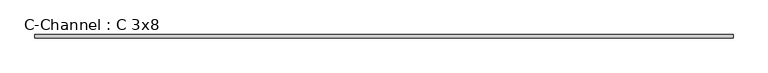
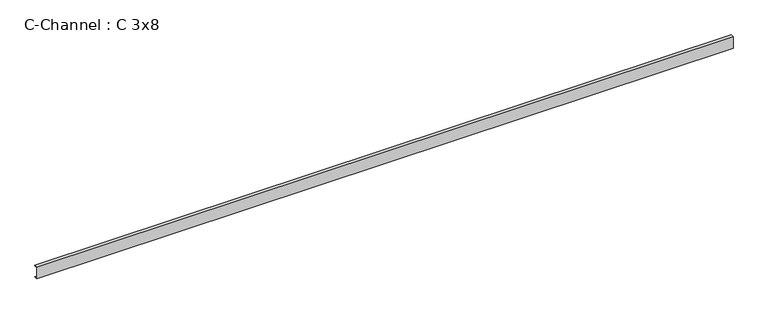
"""IFC4 building model written with IfcOpenShell, lengths in millimetres: beam geometry, C-Channel : C 3x8."""

from ifc_helpers import new_model, si_unit, point, frame, frame_2d, origin, place, context, project, spatial, polyline, circle_curve, trimmed, segment, composite_curve, outline, extrude, source, transform, mapped, element, save


def c_channel_c_3x8_cea8597e(model_context):
    return source(origin(), model_context, "Body", "SweptSolid", [
        extrude(outline(composite_curve([segment(polyline([(-13.5128, 101.6), (44.9072, 101.6)]), True, "CONTINUOUS"), segment(trimmed(circle_curve(frame_2d((35.6108, 101.6)), 9.2964), [point((44.9072, 101.6))], [point((35.6108, 92.3036))], False, "CARTESIAN"), True, "CONTINUOUS"), segment(polyline([(35.6108, 92.3036), (-2.8702, 86.2088084), (-2.8702, -86.2088084), (35.6108, -92.3036)]), True, "CONTINUOUS"), segment(trimmed(circle_curve(frame_2d((35.6108, -101.6)), 9.2964), [point((35.6108, -92.3036))], [point((44.9072, -101.6))], False, "CARTESIAN"), True, "CONTINUOUS"), segment(polyline([(44.9072, -101.6), (-13.5128, -101.6), (-13.5128, 101.6)]), True, "CONTINUOUS")], self_intersect=False)), frame((-5835.65, 0.0, 0.0), z_axis=(1.0, 0.0, 0.0), x_axis=(0.0, 1.0, 0.0)), (0.0, 0.0, 1.0), 11671.3),
    ])


if __name__ == "__main__":
    model = new_model("IFC4")
    model_context = context("Model", 3, world=origin())
    ifc_project = project(units=[si_unit("LENGTHUNIT", "METRE", prefix="MILLI")], contexts=[model_context])
    site = spatial("IfcSite", under=ifc_project)
    building = spatial("IfcBuilding", under=site)
    placement = place(None, origin())
    c_channel_c_3x8_shape = c_channel_c_3x8_cea8597e(model_context)
    element("IfcBeam", 1, ObjectType="C-Channel : C 3x8", at=placement, inside=building, context=model_context, shape_type="MappedRepresentation", body=[
        mapped(c_channel_c_3x8_shape, transform((0.0, 0.0, 0.0), x_axis=(1.0, 0.0, 0.0), y_axis=(0.0, 1.0, 0.0), z_axis=(0.0, 0.0, 1.0))),
    ])
    save(model, "model.ifc")

# Revit data of these elements
# Type "C-Channel : C 3x8"
#   Assembly Code = "B10"
#   W = 14.7
#   Length [instance default] = 5' - 0"
#   bf = 0' - 2.3"
#   d = 0' - 8"
#   tf = 0' - 0.366"
#   tw = 0' - 0.419"
#   x = 0' - 0.532"
#   A = 0.0300694 SF
#   Structural Material [instance default] = Steel ASTM A36
# Element 1 (IfcBeam, "C-Channel : C 3x8")
#   Structural Material = Steel ASTM A992
#   Materials on its faces: "Steel ASTM A992"
# Materials
#   "Steel ASTM A36": class "Metal", colour RGB 199 199 199, transparency 0, Description = "Structural steel, ASTM A36 Grade B, mill finish", Cost = 0
#   "Steel ASTM A992": class "Metal", colour RGB 189 187 185, transparency 0, Description = "Structural steel 50ksi", Cost = 0
